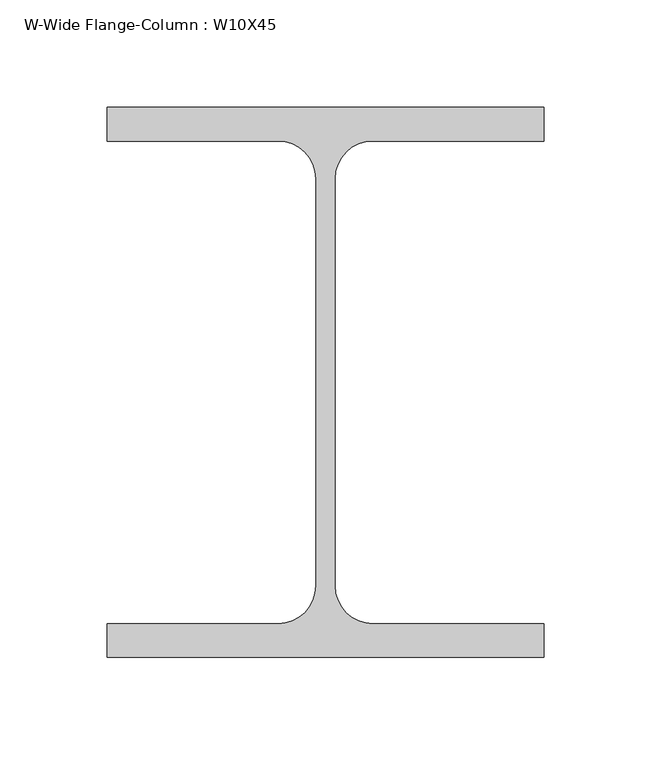
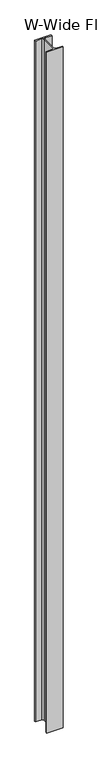
"""IFC4 building model written with IfcOpenShell, lengths in millimetres: column geometry, W-Wide Flange-Column : W10X45."""

import ifcopenshell
import ifcopenshell.guid

model = None  # the IFC model being written
_history = None  # IfcOwnerHistory: only IFC2X3 demands one
_inside = {}  # id of a spatial element -> (the spatial element, [elements in it])
_under = {}  # id of a project, library or spatial element -> (it, [spatial elements below it])
_declared = {}  # id of a project -> (the project, [libraries it declares])
_typed = {}  # id of a type object -> (the type object, [elements of that type])
_made_of = {}  # id of a material, layer set ... -> (it, [elements and type objects made of it])


def new_model(schema):
    """Start an empty IFC model of exactly this schema.

    Asked for "IFC4X3", IfcOpenShell would pick the latest addendum, in which some entities
    have other attributes; the version numbers below select the first issue.
    IFC2X3 requires an IfcOwnerHistory on every rooted entity: one is made here for all.
    """
    global model, _history
    if schema == "IFC4X3":
        model = ifcopenshell.file(schema_version=(4, 3, 0, 0))
    else:
        model = ifcopenshell.file(schema=schema)
    _inside.clear()
    _under.clear()
    _declared.clear()
    _typed.clear()
    _made_of.clear()
    _history = None
    if model.schema == "IFC2X3":
        org = make("IfcOrganization", Name="unknown")
        user = make(
            "IfcPersonAndOrganization",
            ThePerson=make("IfcPerson", FamilyName="unknown"),
            TheOrganization=org,
        )
        app = make(
            "IfcApplication",
            ApplicationDeveloper=org,
            Version="unknown",
            ApplicationFullName="unknown",
            ApplicationIdentifier="unknown",
        )
        _history = make(
            "IfcOwnerHistory",
            OwningUser=user,
            OwningApplication=app,
            ChangeAction="ADDED",
            CreationDate=0,
        )
    return model


def make(cls, **values):
    """One entity of the class cls with the attributes given. An attribute that is None is left unset."""
    return model.create_entity(
        cls, **{name: value for name, value in values.items() if value is not None}
    )


def rooted(cls, **values):
    """An entity with a GlobalId (a new one), such as an element, a storey or a relation."""
    return make(cls, GlobalId=ifcopenshell.guid.new(), OwnerHistory=_history, **values)


def si_unit(unit_type, name, prefix=None):
    """IfcSIUnit, for example si_unit("LENGTHUNIT", "METRE", prefix="MILLI")."""
    return make("IfcSIUnit", UnitType=unit_type, Prefix=prefix, Name=name)


def assignment(units):
    """IfcUnitAssignment: the units of a project."""
    return None if units is None else make("IfcUnitAssignment", Units=units)


def point(xyz):
    """IfcCartesianPoint."""
    return None if xyz is None else make("IfcCartesianPoint", Coordinates=xyz)


def direction(xyz):
    """IfcDirection."""
    return None if xyz is None else make("IfcDirection", DirectionRatios=xyz)


def frame(location, z_axis=None, x_axis=None):
    """IfcAxis2Placement3D, a coordinate frame: its origin and axes. An axis left out is left unset."""
    return make(
        "IfcAxis2Placement3D",
        Location=point(location),
        Axis=direction(z_axis),
        RefDirection=direction(x_axis),
    )


def frame_2d(location, x_axis=None):
    """IfcAxis2Placement2D, a coordinate frame in the plane: its origin and x axis."""
    return make(
        "IfcAxis2Placement2D", Location=point(location), RefDirection=direction(x_axis)
    )


def origin():
    """The frame at (0, 0, 0) with its axes left unset."""
    return frame((0.0, 0.0, 0.0))


def place(relative_to, where):
    """IfcLocalPlacement: puts the frame where relative to a parent placement (None: the world)."""
    return make(
        "IfcLocalPlacement", PlacementRelTo=relative_to, RelativePlacement=where
    )


def context(
    kind, dimensions, precision=None, world=None, true_north=None, identifier=None
):
    """IfcGeometricRepresentationContext, for example the 3D "Model" context."""
    return make(
        "IfcGeometricRepresentationContext",
        ContextIdentifier=identifier,
        ContextType=kind,
        CoordinateSpaceDimension=dimensions,
        Precision=precision,
        WorldCoordinateSystem=world,
        TrueNorth=true_north,
    )


def project(units=None, contexts=None):
    """IfcProject with its units and contexts."""
    return rooted(
        "IfcProject",
        Name="project",
        RepresentationContexts=contexts,
        UnitsInContext=assignment(units),
    )


def spatial(cls, under=None, at=None, **own):
    """A site, building, storey or space (cls), placed at a placement, below another one or the project."""
    s = rooted(cls, ObjectPlacement=at, **own)
    if under is not None:
        _under.setdefault(under.id(), (under, []))[1].append(s)
    return s


def polyline(points):
    """IfcPolyline through the points."""
    return make("IfcPolyline", Points=[point(p) for p in points])


def circle_curve(where, radius):
    """IfcCircle in the frame where."""
    return make("IfcCircle", Position=where, Radius=radius)


def trimmed(basis, trim1, trim2, sense, master):
    """IfcTrimmedCurve: the piece of a basis curve between two trims."""
    return make(
        "IfcTrimmedCurve",
        BasisCurve=basis,
        Trim1=trim1,
        Trim2=trim2,
        SenseAgreement=sense,
        MasterRepresentation=master,
    )


def segment(curve, same_sense, transition):
    """IfcCompositeCurveSegment."""
    return make(
        "IfcCompositeCurveSegment",
        Transition=transition,
        SameSense=same_sense,
        ParentCurve=curve,
    )


def composite_curve(segments, self_intersect=None):
    """IfcCompositeCurve: segments joined end to end."""
    return make("IfcCompositeCurve", Segments=segments, SelfIntersect=self_intersect)


def outline(outer, holes=None, kind="AREA"):
    """IfcArbitraryClosedProfileDef: a profile drawn as a closed curve; with holes, ...WithVoids."""
    if holes is None:
        return make("IfcArbitraryClosedProfileDef", ProfileType=kind, OuterCurve=outer)
    return make(
        "IfcArbitraryProfileDefWithVoids",
        ProfileType=kind,
        OuterCurve=outer,
        InnerCurves=holes,
    )


def extrude(swept, where, along, depth):
    """IfcExtrudedAreaSolid: the profile swept, set in the frame where, extruded along a direction by depth."""
    return make(
        "IfcExtrudedAreaSolid",
        SweptArea=swept,
        Position=where,
        ExtrudedDirection=direction(along),
        Depth=depth,
    )


def shape(context_of_items, identifier, shape_type, items):
    """IfcShapeRepresentation: the items that make up one representation, for example the "Body"."""
    return make(
        "IfcShapeRepresentation",
        ContextOfItems=context_of_items,
        RepresentationIdentifier=identifier,
        RepresentationType=shape_type,
        Items=items,
    )


def source(mapping_origin, context_of_items, identifier, shape_type, items):
    """IfcRepresentationMap: a shape defined once, which mapped items show again and again."""
    return make(
        "IfcRepresentationMap",
        MappingOrigin=mapping_origin,
        MappedRepresentation=shape(context_of_items, identifier, shape_type, items),
    )


def transform(
    local_origin,
    x_axis=None,
    y_axis=None,
    z_axis=None,
    scale=None,
    scale2=None,
    scale3=None,
    uniform=True,
):
    """IfcCartesianTransformationOperator3D, or its non-uniform kind. x_axis, y_axis, z_axis: its Axis1, 2, 3."""
    if uniform:
        return make(
            "IfcCartesianTransformationOperator3D",
            Axis1=direction(x_axis),
            Axis2=direction(y_axis),
            LocalOrigin=point(local_origin),
            Scale=scale,
            Axis3=direction(z_axis),
        )
    return make(
        "IfcCartesianTransformationOperator3DnonUniform",
        Axis1=direction(x_axis),
        Axis2=direction(y_axis),
        LocalOrigin=point(local_origin),
        Scale=scale,
        Axis3=direction(z_axis),
        Scale2=scale2,
        Scale3=scale3,
    )


def mapped(mapping_source, mapping_target):
    """IfcMappedItem: shows the shape of a source again, moved by a transform."""
    return make(
        "IfcMappedItem", MappingSource=mapping_source, MappingTarget=mapping_target
    )


def made_of(thing, what):
    """Note that an element or type object is made of a material, layer set ...; save() writes the relation."""
    if what is not None:
        _made_of.setdefault(what.id(), (what, []))[1].append(thing)
    return thing


def element(
    cls,
    number,
    at=None,
    inside=None,
    cuts=None,
    type_object=None,
    material=None,
    context=None,
    identifier="Body",
    shape_type=None,
    held_by="IfcProductDefinitionShape",
    body=None,
    shapes=None,
    **own,
):
    """One element of the class cls, such as IfcWall. Its Tag is "e" and its number.

    at: its placement. inside: the storey or other place that contains it. cuts: it is an
    opening in that element (IfcRelVoidsElement). A single representation is given by context,
    identifier, shape_type and body (its items); several are given by shapes. held_by: the class
    of the entity that holds the representations. save() writes the other relations.
    """
    e = rooted(cls, Tag="e%d" % number, ObjectPlacement=at, **own)
    if body is not None:
        shapes = [shape(context, identifier, shape_type, body)]
    if shapes is not None:
        e.Representation = make(held_by, Representations=shapes)
    if inside is not None:
        _inside.setdefault(inside.id(), (inside, []))[1].append(e)
    if cuts is not None:
        rooted(
            "IfcRelVoidsElement", RelatingBuildingElement=cuts, RelatedOpeningElement=e
        )
    if type_object is not None:
        _typed.setdefault(type_object.id(), (type_object, []))[1].append(e)
    return made_of(e, material)


def aggregate(whole, parts):
    """IfcRelAggregates: a whole, such as a stair, and the parts it consists of."""
    return rooted("IfcRelAggregates", RelatingObject=whole, RelatedObjects=parts)


def save(model, path):
    """Write the relations noted so far, then the file.

    IfcRelAggregates (storeys below a building ...), IfcRelContainedInSpatialStructure (elements
    in a storey), IfcRelDefinesByType, IfcRelAssociatesMaterial and IfcRelDeclares: one each for
    every whole, place, type object, material and project.
    """
    for whole, parts in _under.values():
        aggregate(whole, parts)
    for where, things in _inside.values():
        rooted(
            "IfcRelContainedInSpatialStructure",
            RelatedElements=things,
            RelatingStructure=where,
        )
    for kind, things in _typed.values():
        rooted("IfcRelDefinesByType", RelatedObjects=things, RelatingType=kind)
    for what, things in _made_of.values():
        rooted("IfcRelAssociatesMaterial", RelatedObjects=things, RelatingMaterial=what)
    for by, libraries in _declared.values():
        rooted("IfcRelDeclares", RelatingContext=by, RelatedDefinitions=libraries)
    model.write(path)


def w_wide_flange_column_w10x45_18ccb682(model_context):
    return source(origin(), model_context, "Body", "SweptSolid", [
        extrude(outline(composite_curve([segment(polyline([(101.854, 128.27), (101.854, 112.522), (22.0345, 112.522)]), True, "CONTINUOUS"), segment(trimmed(circle_curve(frame_2d((22.0345, 94.9325)), 17.5895), [point((22.0345, 112.522))], [point((4.445, 94.9325))], True, "CARTESIAN"), True, "CONTINUOUS"), segment(polyline([(4.445, 94.9325), (4.445, -94.9325)]), True, "CONTINUOUS"), segment(trimmed(circle_curve(frame_2d((22.0345, -94.9325)), 17.5895), [point((4.445, -94.9325))], [point((22.0345, -112.522))], True, "CARTESIAN"), True, "CONTINUOUS"), segment(polyline([(22.0345, -112.522), (101.854, -112.522), (101.854, -128.27), (-101.854, -128.27), (-101.854, -112.522), (-22.0345, -112.522)]), True, "CONTINUOUS"), segment(trimmed(circle_curve(frame_2d((-22.0345, -94.9325)), 17.5895), [point((-22.0345, -112.522))], [point((-4.445, -94.9325))], True, "CARTESIAN"), True, "CONTINUOUS"), segment(polyline([(-4.445, -94.9325), (-4.445, 94.9325)]), True, "CONTINUOUS"), segment(trimmed(circle_curve(frame_2d((-22.0345, 94.9325)), 17.5895), [point((-4.445, 94.9325))], [point((-22.0345, 112.522))], True, "CARTESIAN"), True, "CONTINUOUS"), segment(polyline([(-22.0345, 112.522), (-101.854, 112.522), (-101.854, 128.27), (101.854, 128.27)]), True, "CONTINUOUS")], self_intersect=False)), frame((0.0, 0.0, 8756.65), z_axis=(0.0, 0.0, 1.0), x_axis=(1.0, 0.0, 0.0)), (0.0, 0.0, 1.0), 8870.95),
    ])


if __name__ == "__main__":
    model = new_model("IFC4")
    model_context = context("Model", 3, world=origin())
    ifc_project = project(units=[si_unit("LENGTHUNIT", "METRE", prefix="MILLI")], contexts=[model_context])
    site = spatial("IfcSite", under=ifc_project)
    building = spatial("IfcBuilding", under=site)
    placement = place(None, origin())
    w_wide_flange_column_w10x45_shape = w_wide_flange_column_w10x45_18ccb682(model_context)
    element("IfcColumn", 1, ObjectType="W-Wide Flange-Column : W10X45", at=placement, inside=building, context=model_context, shape_type="MappedRepresentation", body=[
        mapped(w_wide_flange_column_w10x45_shape, transform((0.0, 0.0, 0.0), x_axis=(1.0, 0.0, 0.0), y_axis=(0.0, 1.0, 0.0), z_axis=(0.0, 0.0, 1.0))),
    ])
    save(model, "model.ifc")

# Revit data of these elements
# Type "W-Wide Flange-Column : W10X45"
#   Assembly Code = "B10"
#   W = 45
#   bf = 0' - 8.02"
#   d = 0' - 10.1"
#   k = 0' - 1 5/16"
#   kr = 0' - 0.6925"
#   tf = 0' - 0.62"
#   tw = 0' - 0.35"
#   A = 0.0923611 SF
#   Structural Material [instance default] = Steel ASTM A992
# Element 1 (IfcColumn, "W-Wide Flange-Column : W10X45")
#   Materials on its faces: "Steel ASTM A992"
# Materials
#   "Steel ASTM A992": class "Metal", colour RGB 199 199 199, transparency 0, Description = "Structural steel 50ksi", Cost = 0
